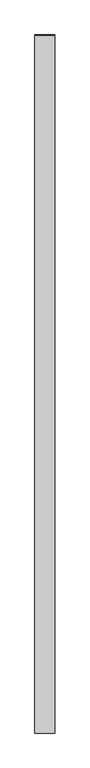
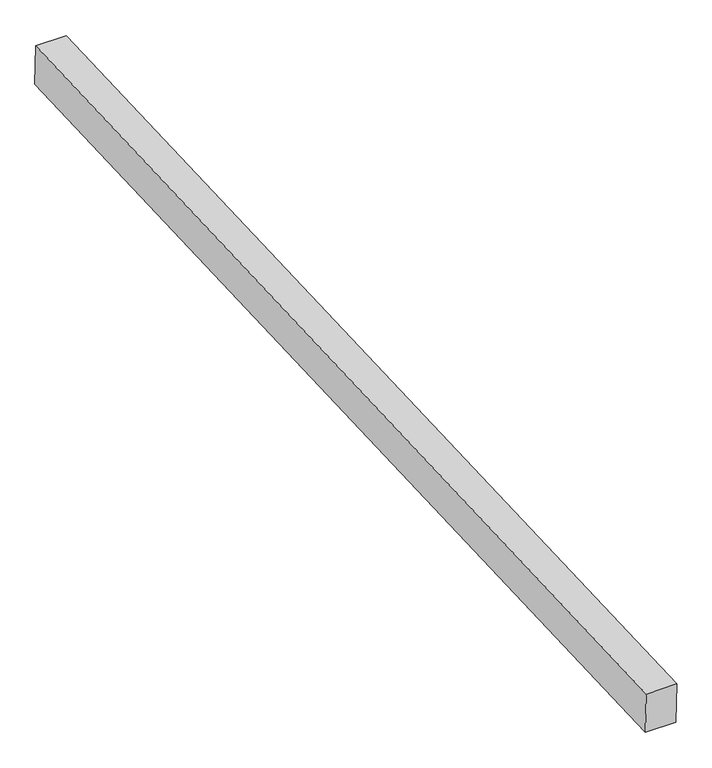
"""IFC4 building model written with IfcOpenShell, lengths in millimetres: proxy geometry, Generic Models 7:Generic Models 1:8:Generic Models 1:8 : Generic Models 7:Generic Models 1:337419:51 : Generic Models 7:Generic Models 1:8:Generic Models 1:8 : Generic Models 7:Generic Models 1:337419:315935."""

from ifc_helpers import new_model, si_unit, frame, origin, place, context, project, spatial, polyline, outline, extrude, source, transform, mapped, element, save


def generic_models_c4bff049(model_context):
    return source(origin(), model_context, "Body", "SweptSolid", [
        extrude(outline(polyline([(-581229.2495411, 3818.908703), (-576356.3266468, 4021.9471569), (-576348.7597251, 3831.5971524), (-581221.3189223, 3628.5738526), (-581229.2495411, 3818.908703)])), frame((610822.761724, 0.0, 0.0), z_axis=(1.0, 0.0, 0.0), x_axis=(0.0, 1.0, 0.0)), (0.0, 0.0, 1.0), 139.7),
    ])


if __name__ == "__main__":
    model = new_model("IFC4")
    model_context = context("Model", 3, world=origin())
    ifc_project = project(units=[si_unit("LENGTHUNIT", "METRE", prefix="MILLI")], contexts=[model_context])
    site = spatial("IfcSite", under=ifc_project)
    building = spatial("IfcBuilding", under=site)
    placement = place(None, origin())
    generic_models_shape = generic_models_c4bff049(model_context)
    element("IfcBuildingElementProxy", 1, Name="Generic Models 7:Generic Models 1:8:Generic Models 1:8 : Generic Models 7:Generic Models 1:337419:51 : Generic Models 7:Generic Models 1:8:Generic Models 1:8 : Generic Models 7:Generic Models 1:337419:315935", ObjectType="Generic Models 7:Generic Models 1:8:Generic Models 1:8 : Generic Models 7:Generic Models 1:337419:51 : Generic Models 7:Generic Models 1:8:Generic Models 1:8 : Generic Models 7:Generic Models 1:337419:315935", at=placement, inside=building, context=model_context, shape_type="MappedRepresentation", body=[
        mapped(generic_models_shape, transform((0.0, 0.0, 0.0), x_axis=(1.0, 0.0, 0.0), y_axis=(0.0, 1.0, 0.0), z_axis=(0.0, 0.0, 1.0))),
    ])
    save(model, "model.ifc")

# Revit data of these elements
# Type "Generic Models 7:Generic Models 1:8:Generic Models 1:8 : Generic Models 7:Generic Models 1:337419:51 : Generic Models 7:Generic Models 1:8:Generic Models 1:8 : Generic Models 7:Generic Models 1:337419:315935"
#   NameOverride = "Generic Models 7:Generic Models 1:8:Generic Models 1:8 : Generic Models 7:Generic Models 1:337419:315935"
#   ObjectTypeOverride = "Generic Models 1:8 : Generic Models 7:Generic Models 1:337419"
#   Reference = "Generic Models 1"
#   Tag = "315935"
# Element 1 (IfcBuildingElementProxy, "Generic Models 7:Generic Models 1:8:Generic Models 1:8 : Generic Models 7:Generic Models 1:337419:51 : Generic Models 7:Generic Models 1:8:Generic Models 1:8 : Generic Models 7:Generic Models 1:337419:315935")
#   Materials on its faces: "5 1/2\" X 7 1/2\" EXTERIOR GRADE GLULAM BEAMS"
# Materials
#   "5 1/2\" X 7 1/2\" EXTERIOR GRADE GLULAM BEAMS": class "Wood", colour RGB 183 134 68, transparency 0, Keynote = "M06181300.01", Description = "Pinus Echinata", Cost = 0
